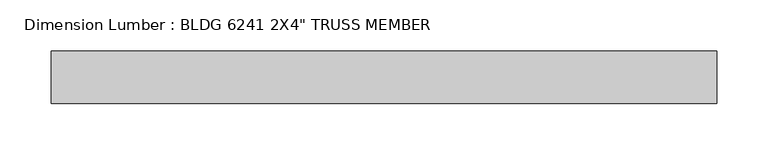
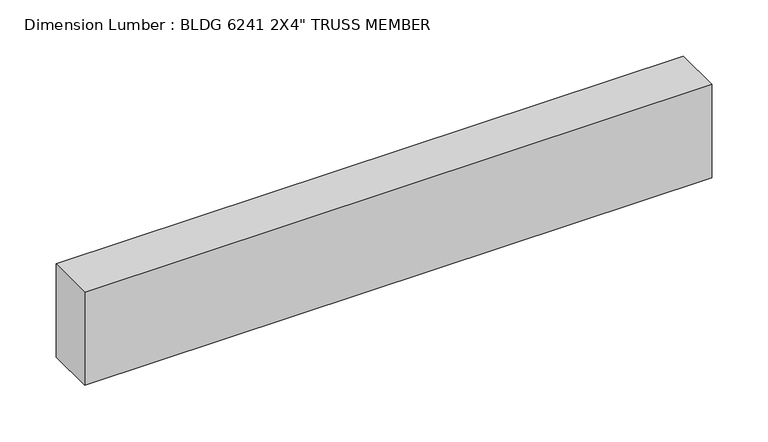
"""IFC4 building model written with IfcOpenShell, lengths in millimetres: beam geometry."""

from ifc_helpers import new_model, si_unit, frame, origin, place, context, project, spatial, polyline, outline, extrude, source, transform, mapped, element, save


def beam_99e5442a(model_context):
    return source(origin(), model_context, "Body", "SweptSolid", [
        extrude(outline(polyline([(350.5042173, -25.4), (-295.4519367, -25.4), (-295.4519367, 25.4), (350.5042173, 25.4), (350.5042173, -25.4)])), frame((0.0, 0.0, -50.8), z_axis=(0.0, 0.0, 1.0), x_axis=(1.0, 0.0, 0.0)), (0.0, 0.0, 1.0), 101.6),
    ])


if __name__ == "__main__":
    model = new_model("IFC4")
    model_context = context("Model", 3, world=origin())
    ifc_project = project(units=[si_unit("LENGTHUNIT", "METRE", prefix="MILLI")], contexts=[model_context])
    site = spatial("IfcSite", under=ifc_project)
    building = spatial("IfcBuilding", under=site)
    placement = place(None, origin())
    beam_shape = beam_99e5442a(model_context)
    element("IfcBeam", 1, ObjectType="Dimension Lumber : BLDG 6241 2X4\" TRUSS MEMBER", at=placement, inside=building, context=model_context, shape_type="MappedRepresentation", body=[
        mapped(beam_shape, transform((0.0, 0.0, 0.0), x_axis=(1.0, 0.0, 0.0), y_axis=(0.0, 1.0, 0.0), z_axis=(0.0, 0.0, 1.0))),
    ])
    save(model, "model.ifc")

# Revit data of these elements
# Type "Dimension Lumber : BLDG 6241 2X4\" TRUSS MEMBER"
#   Assembly Code = "B10"
#   A = 0.273472 SF
#   Length [instance default] = 5' - 0"
#   b = 0' - 2"
#   d = 0' - 4"
#   Structural Material [instance default] = Softwood, Lumber
# Element 1 (IfcBeam, "Dimension Lumber : BLDG 6241 2X4\" TRUSS MEMBER")
#   Materials on its faces: "Softwood, Lumber"
# Materials
#   "Softwood, Lumber": class "Wood", colour RGB 223 192 134, transparency 0, Description = "Pinus Echinata", Cost = 0
